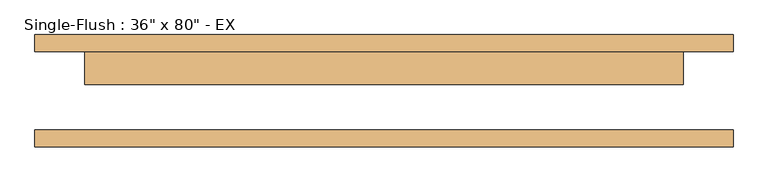
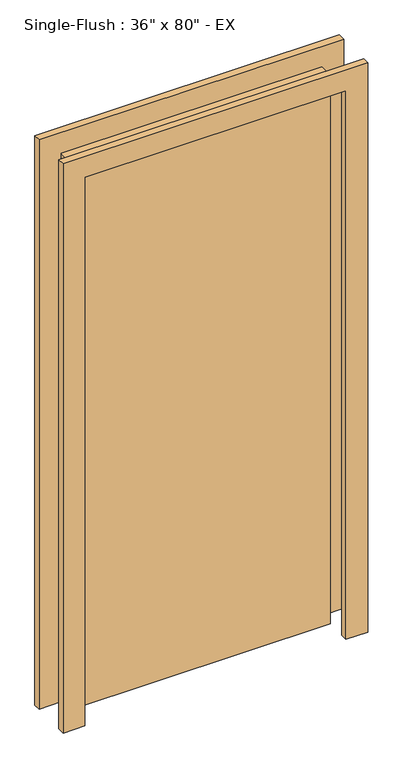
"""IFC4 building model written with IfcOpenShell, lengths in millimetres: door geometry."""

from ifc_helpers import new_model, si_unit, frame, origin, origin_with_axes, place, context, project, spatial, polyline, outline, extrude, source, transform, mapped, element, save


def door_156d4006(model_context):
    return source(origin(), model_context, "Body", "SweptSolid", [
        extrude(outline(polyline([(2108.2, -533.4), (0.0, -533.4), (0.0, -457.2), (2032.0, -457.2), (2032.0, 457.2), (0.0, 457.2), (0.0, 533.4), (2108.2, 533.4), (2108.2, -533.4)])), frame((0.0, 60.325, 0.0), z_axis=(0.0, 1.0, 0.0), x_axis=(0.0, 0.0, 1.0)), (0.0, 0.0, 1.0), 25.4),
        extrude(outline(polyline([(2108.2, 533.4), (2108.2, -533.4), (0.0, -533.4), (0.0, -457.2), (2032.0, -457.2), (2032.0, 457.2), (0.0, 457.2), (0.0, 533.4), (2108.2, 533.4)])), frame((0.0, -85.725, 0.0), z_axis=(0.0, 1.0, 0.0), x_axis=(0.0, 0.0, 1.0)), (0.0, 0.0, 1.0), 25.4),
        extrude(outline(polyline([(457.2, 9.525), (-457.2, 9.525), (-457.2, 60.325), (457.2, 60.325), (457.2, 9.525)])), origin_with_axes(), (0.0, 0.0, 1.0), 2032.0),
    ])


if __name__ == "__main__":
    model = new_model("IFC4")
    model_context = context("Model", 3, world=origin())
    ifc_project = project(units=[si_unit("LENGTHUNIT", "METRE", prefix="MILLI")], contexts=[model_context])
    site = spatial("IfcSite", under=ifc_project)
    building = spatial("IfcBuilding", under=site)
    placement = place(None, origin())
    door_shape = door_156d4006(model_context)
    element("IfcDoor", 1, ObjectType="Single-Flush : 36\" x 80\" - EX", at=placement, inside=building, context=model_context, shape_type="MappedRepresentation", body=[
        mapped(door_shape, transform((0.0, 0.0, 0.0), x_axis=(1.0, 0.0, 0.0), y_axis=(0.0, 1.0, 0.0), z_axis=(0.0, 0.0, 1.0))),
    ])
    save(model, "model.ifc")

# Revit data of these elements
# Type "Single-Flush : 36\" x 80\" - EX"
#   Type Mark = "EX-2"
#   Fire_Rating = ""
#   Assembly Code = "C1020"
#   Thickness = 0' - 2"
#   Height = 6' - 8"
#   Trim Projection Ext = 0' - 1"
#   Trim Projection Int = 0' - 1"
#   Trim Width = 0' - 3"
#   Width = 3' - 0"
#   Door Material = drywall
#   Frame Material = drywall
#   Function = (empty or 0)
#   Wall Closure = (empty or 0)
# Element 1 (IfcDoor, "Single-Flush : 36\" x 80\" - EX")
#   Materials on its faces: "drywall"
# Materials
#   "drywall": class "Generic", colour RGB 255 255 255, transparency 0, Description = "Gypsum Wall Board", Cost = 0
